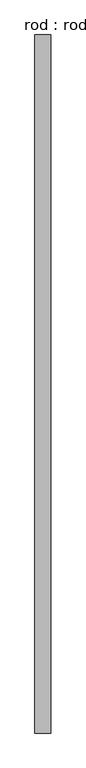
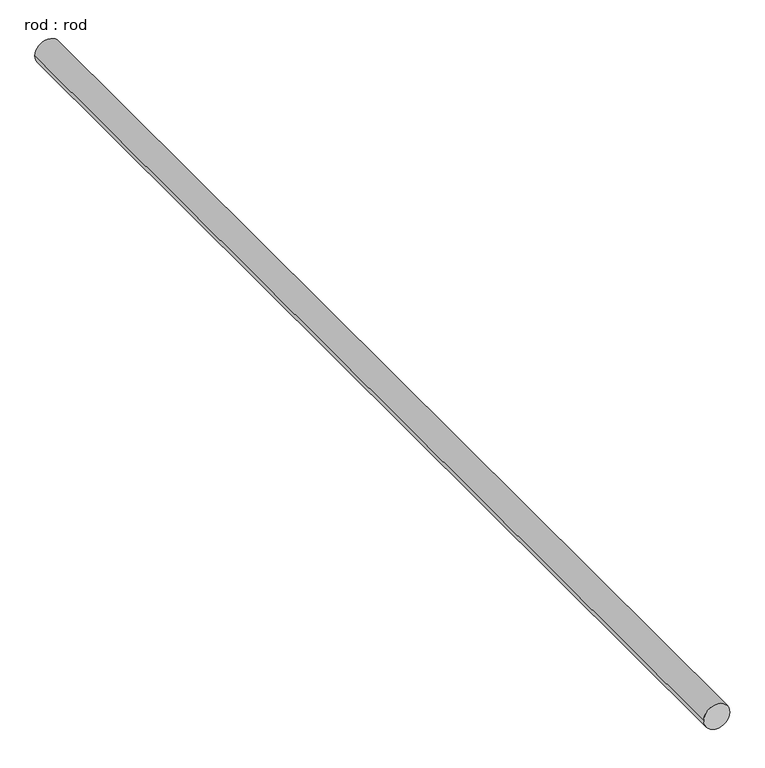
"""IFC4 building model written with IfcOpenShell, lengths in millimetres: proxy geometry, rod : rod."""

import ifcopenshell
import ifcopenshell.guid

model = None  # the IFC model being written
_history = None  # IfcOwnerHistory: only IFC2X3 demands one
_inside = {}  # id of a spatial element -> (the spatial element, [elements in it])
_under = {}  # id of a project, library or spatial element -> (it, [spatial elements below it])
_declared = {}  # id of a project -> (the project, [libraries it declares])
_typed = {}  # id of a type object -> (the type object, [elements of that type])
_made_of = {}  # id of a material, layer set ... -> (it, [elements and type objects made of it])


def new_model(schema):
    """Start an empty IFC model of exactly this schema.

    Asked for "IFC4X3", IfcOpenShell would pick the latest addendum, in which some entities
    have other attributes; the version numbers below select the first issue.
    IFC2X3 requires an IfcOwnerHistory on every rooted entity: one is made here for all.
    """
    global model, _history
    if schema == "IFC4X3":
        model = ifcopenshell.file(schema_version=(4, 3, 0, 0))
    else:
        model = ifcopenshell.file(schema=schema)
    _inside.clear()
    _under.clear()
    _declared.clear()
    _typed.clear()
    _made_of.clear()
    _history = None
    if model.schema == "IFC2X3":
        org = make("IfcOrganization", Name="unknown")
        user = make(
            "IfcPersonAndOrganization",
            ThePerson=make("IfcPerson", FamilyName="unknown"),
            TheOrganization=org,
        )
        app = make(
            "IfcApplication",
            ApplicationDeveloper=org,
            Version="unknown",
            ApplicationFullName="unknown",
            ApplicationIdentifier="unknown",
        )
        _history = make(
            "IfcOwnerHistory",
            OwningUser=user,
            OwningApplication=app,
            ChangeAction="ADDED",
            CreationDate=0,
        )
    return model


def make(cls, **values):
    """One entity of the class cls with the attributes given. An attribute that is None is left unset."""
    return model.create_entity(
        cls, **{name: value for name, value in values.items() if value is not None}
    )


def rooted(cls, **values):
    """An entity with a GlobalId (a new one), such as an element, a storey or a relation."""
    return make(cls, GlobalId=ifcopenshell.guid.new(), OwnerHistory=_history, **values)


def si_unit(unit_type, name, prefix=None):
    """IfcSIUnit, for example si_unit("LENGTHUNIT", "METRE", prefix="MILLI")."""
    return make("IfcSIUnit", UnitType=unit_type, Prefix=prefix, Name=name)


def assignment(units):
    """IfcUnitAssignment: the units of a project."""
    return None if units is None else make("IfcUnitAssignment", Units=units)


def point(xyz):
    """IfcCartesianPoint."""
    return None if xyz is None else make("IfcCartesianPoint", Coordinates=xyz)


def direction(xyz):
    """IfcDirection."""
    return None if xyz is None else make("IfcDirection", DirectionRatios=xyz)


def frame(location, z_axis=None, x_axis=None):
    """IfcAxis2Placement3D, a coordinate frame: its origin and axes. An axis left out is left unset."""
    return make(
        "IfcAxis2Placement3D",
        Location=point(location),
        Axis=direction(z_axis),
        RefDirection=direction(x_axis),
    )


def frame_2d(location, x_axis=None):
    """IfcAxis2Placement2D, a coordinate frame in the plane: its origin and x axis."""
    return make(
        "IfcAxis2Placement2D", Location=point(location), RefDirection=direction(x_axis)
    )


def origin():
    """The frame at (0, 0, 0) with its axes left unset."""
    return frame((0.0, 0.0, 0.0))


def place(relative_to, where):
    """IfcLocalPlacement: puts the frame where relative to a parent placement (None: the world)."""
    return make(
        "IfcLocalPlacement", PlacementRelTo=relative_to, RelativePlacement=where
    )


def context(
    kind, dimensions, precision=None, world=None, true_north=None, identifier=None
):
    """IfcGeometricRepresentationContext, for example the 3D "Model" context."""
    return make(
        "IfcGeometricRepresentationContext",
        ContextIdentifier=identifier,
        ContextType=kind,
        CoordinateSpaceDimension=dimensions,
        Precision=precision,
        WorldCoordinateSystem=world,
        TrueNorth=true_north,
    )


def project(units=None, contexts=None):
    """IfcProject with its units and contexts."""
    return rooted(
        "IfcProject",
        Name="project",
        RepresentationContexts=contexts,
        UnitsInContext=assignment(units),
    )


def spatial(cls, under=None, at=None, **own):
    """A site, building, storey or space (cls), placed at a placement, below another one or the project."""
    s = rooted(cls, ObjectPlacement=at, **own)
    if under is not None:
        _under.setdefault(under.id(), (under, []))[1].append(s)
    return s


def circle_curve(where, radius):
    """IfcCircle in the frame where."""
    return make("IfcCircle", Position=where, Radius=radius)


def trimmed(basis, trim1, trim2, sense, master):
    """IfcTrimmedCurve: the piece of a basis curve between two trims."""
    return make(
        "IfcTrimmedCurve",
        BasisCurve=basis,
        Trim1=trim1,
        Trim2=trim2,
        SenseAgreement=sense,
        MasterRepresentation=master,
    )


def segment(curve, same_sense, transition):
    """IfcCompositeCurveSegment."""
    return make(
        "IfcCompositeCurveSegment",
        Transition=transition,
        SameSense=same_sense,
        ParentCurve=curve,
    )


def composite_curve(segments, self_intersect=None):
    """IfcCompositeCurve: segments joined end to end."""
    return make("IfcCompositeCurve", Segments=segments, SelfIntersect=self_intersect)


def outline(outer, holes=None, kind="AREA"):
    """IfcArbitraryClosedProfileDef: a profile drawn as a closed curve; with holes, ...WithVoids."""
    if holes is None:
        return make("IfcArbitraryClosedProfileDef", ProfileType=kind, OuterCurve=outer)
    return make(
        "IfcArbitraryProfileDefWithVoids",
        ProfileType=kind,
        OuterCurve=outer,
        InnerCurves=holes,
    )


def extrude(swept, where, along, depth):
    """IfcExtrudedAreaSolid: the profile swept, set in the frame where, extruded along a direction by depth."""
    return make(
        "IfcExtrudedAreaSolid",
        SweptArea=swept,
        Position=where,
        ExtrudedDirection=direction(along),
        Depth=depth,
    )


def shape(context_of_items, identifier, shape_type, items):
    """IfcShapeRepresentation: the items that make up one representation, for example the "Body"."""
    return make(
        "IfcShapeRepresentation",
        ContextOfItems=context_of_items,
        RepresentationIdentifier=identifier,
        RepresentationType=shape_type,
        Items=items,
    )


def source(mapping_origin, context_of_items, identifier, shape_type, items):
    """IfcRepresentationMap: a shape defined once, which mapped items show again and again."""
    return make(
        "IfcRepresentationMap",
        MappingOrigin=mapping_origin,
        MappedRepresentation=shape(context_of_items, identifier, shape_type, items),
    )


def transform(
    local_origin,
    x_axis=None,
    y_axis=None,
    z_axis=None,
    scale=None,
    scale2=None,
    scale3=None,
    uniform=True,
):
    """IfcCartesianTransformationOperator3D, or its non-uniform kind. x_axis, y_axis, z_axis: its Axis1, 2, 3."""
    if uniform:
        return make(
            "IfcCartesianTransformationOperator3D",
            Axis1=direction(x_axis),
            Axis2=direction(y_axis),
            LocalOrigin=point(local_origin),
            Scale=scale,
            Axis3=direction(z_axis),
        )
    return make(
        "IfcCartesianTransformationOperator3DnonUniform",
        Axis1=direction(x_axis),
        Axis2=direction(y_axis),
        LocalOrigin=point(local_origin),
        Scale=scale,
        Axis3=direction(z_axis),
        Scale2=scale2,
        Scale3=scale3,
    )


def mapped(mapping_source, mapping_target):
    """IfcMappedItem: shows the shape of a source again, moved by a transform."""
    return make(
        "IfcMappedItem", MappingSource=mapping_source, MappingTarget=mapping_target
    )


def made_of(thing, what):
    """Note that an element or type object is made of a material, layer set ...; save() writes the relation."""
    if what is not None:
        _made_of.setdefault(what.id(), (what, []))[1].append(thing)
    return thing


def element(
    cls,
    number,
    at=None,
    inside=None,
    cuts=None,
    type_object=None,
    material=None,
    context=None,
    identifier="Body",
    shape_type=None,
    held_by="IfcProductDefinitionShape",
    body=None,
    shapes=None,
    **own,
):
    """One element of the class cls, such as IfcWall. Its Tag is "e" and its number.

    at: its placement. inside: the storey or other place that contains it. cuts: it is an
    opening in that element (IfcRelVoidsElement). A single representation is given by context,
    identifier, shape_type and body (its items); several are given by shapes. held_by: the class
    of the entity that holds the representations. save() writes the other relations.
    """
    e = rooted(cls, Tag="e%d" % number, ObjectPlacement=at, **own)
    if body is not None:
        shapes = [shape(context, identifier, shape_type, body)]
    if shapes is not None:
        e.Representation = make(held_by, Representations=shapes)
    if inside is not None:
        _inside.setdefault(inside.id(), (inside, []))[1].append(e)
    if cuts is not None:
        rooted(
            "IfcRelVoidsElement", RelatingBuildingElement=cuts, RelatedOpeningElement=e
        )
    if type_object is not None:
        _typed.setdefault(type_object.id(), (type_object, []))[1].append(e)
    return made_of(e, material)


def aggregate(whole, parts):
    """IfcRelAggregates: a whole, such as a stair, and the parts it consists of."""
    return rooted("IfcRelAggregates", RelatingObject=whole, RelatedObjects=parts)


def save(model, path):
    """Write the relations noted so far, then the file.

    IfcRelAggregates (storeys below a building ...), IfcRelContainedInSpatialStructure (elements
    in a storey), IfcRelDefinesByType, IfcRelAssociatesMaterial and IfcRelDeclares: one each for
    every whole, place, type object, material and project.
    """
    for whole, parts in _under.values():
        aggregate(whole, parts)
    for where, things in _inside.values():
        rooted(
            "IfcRelContainedInSpatialStructure",
            RelatedElements=things,
            RelatingStructure=where,
        )
    for kind, things in _typed.values():
        rooted("IfcRelDefinesByType", RelatedObjects=things, RelatingType=kind)
    for what, things in _made_of.values():
        rooted("IfcRelAssociatesMaterial", RelatedObjects=things, RelatingMaterial=what)
    for by, libraries in _declared.values():
        rooted("IfcRelDeclares", RelatingContext=by, RelatedDefinitions=libraries)
    model.write(path)


def rod_rod_be3269fa(model_context):
    return source(origin(), model_context, "Body", "SweptSolid", [
        extrude(outline(composite_curve([segment(trimmed(circle_curve(frame_2d((0.0108462, 0.0)), 200.0), [point((0.0108462, 200.0))], [point((0.0108462, -200.0))], False, "CARTESIAN"), True, "CONTINUOUS"), segment(trimmed(circle_curve(frame_2d((0.0108462, 0.0)), 200.0), [point((0.0108462, -200.0))], [point((0.0108462, 200.0))], False, "CARTESIAN"), True, "CONTINUOUS")], self_intersect=False)), frame((0.0, -4782.2713847, 0.0), z_axis=(0.0, 1.0, 0.0), x_axis=(0.0, 0.0, 1.0)), (0.0, 0.0, 1.0), 17750.0),
    ])


if __name__ == "__main__":
    model = new_model("IFC4")
    model_context = context("Model", 3, world=origin())
    ifc_project = project(units=[si_unit("LENGTHUNIT", "METRE", prefix="MILLI")], contexts=[model_context])
    site = spatial("IfcSite", under=ifc_project)
    building = spatial("IfcBuilding", under=site)
    placement = place(None, origin())
    rod_rod_shape = rod_rod_be3269fa(model_context)
    element("IfcBuildingElementProxy", 1, Name="rod : rod", ObjectType="rod : rod", at=placement, inside=building, context=model_context, shape_type="MappedRepresentation", body=[
        mapped(rod_rod_shape, transform((0.0, 0.0, 0.0), x_axis=(1.0, 0.0, 0.0), y_axis=(0.0, 1.0, 0.0), z_axis=(0.0, 0.0, 1.0))),
    ])
    save(model, "model.ifc")

# Revit data of these elements
# Type "rod : rod"
#   Default Elevation = 0
